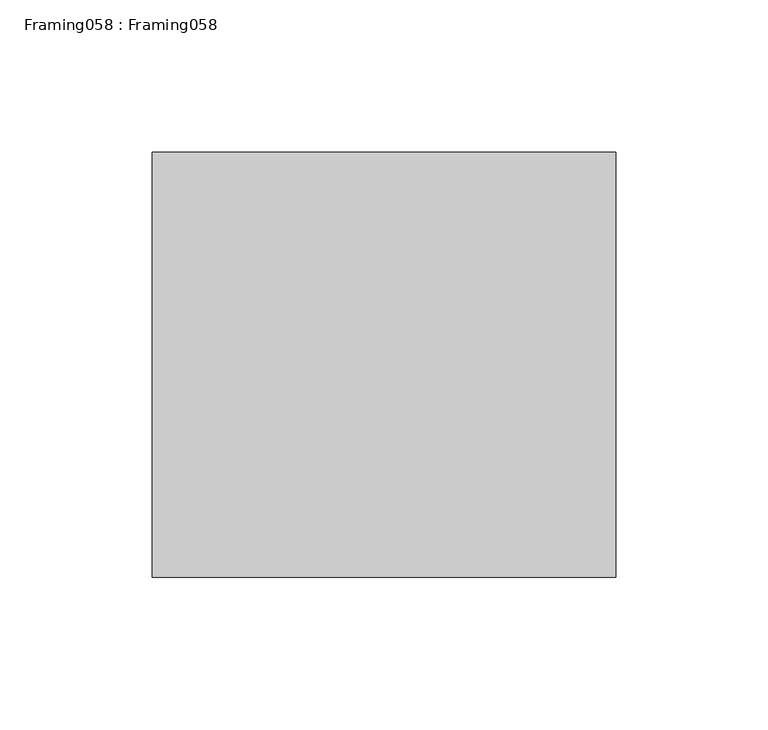
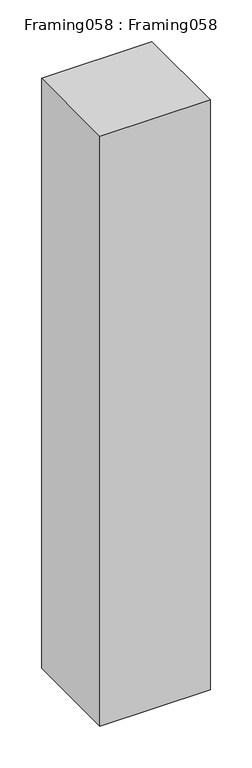
"""IFC4 building model written with IfcOpenShell, lengths in millimetres: proxy geometry, Framing058 : Framing058."""

from ifc_helpers import new_model, si_unit, frame, origin, place, context, project, spatial, polyline, outline, extrude, source, transform, mapped, element, save


def framing058_framing058_3deb3078(model_context):
    return source(origin(), model_context, "Body", "SweptSolid", [
        extrude(outline(polyline([(4475.0880859, 9730.3383229), (4475.0880859, 9590.6375834), (4322.6880859, 9590.6375834), (4322.6880859, 9730.3383229), (4475.0880859, 9730.3383229)])), frame((0.0, 0.0, 36582.096), z_axis=(0.0, 0.0, 1.0), x_axis=(1.0, 0.0, 0.0)), (0.0, 0.0, 1.0), 863.6),
    ])


if __name__ == "__main__":
    model = new_model("IFC4")
    model_context = context("Model", 3, world=origin())
    ifc_project = project(units=[si_unit("LENGTHUNIT", "METRE", prefix="MILLI")], contexts=[model_context])
    site = spatial("IfcSite", under=ifc_project)
    building = spatial("IfcBuilding", under=site)
    placement = place(None, origin())
    framing058_framing058_shape = framing058_framing058_3deb3078(model_context)
    element("IfcBuildingElementProxy", 1, Name="Framing058 : Framing058", ObjectType="Framing058 : Framing058", at=placement, inside=building, context=model_context, shape_type="MappedRepresentation", body=[
        mapped(framing058_framing058_shape, transform((0.0, 0.0, 0.0), x_axis=(1.0, 0.0, 0.0), y_axis=(0.0, 1.0, 0.0), z_axis=(0.0, 0.0, 1.0))),
    ])
    save(model, "model.ifc")

# Revit data of these elements
# Type "Framing058 : Framing058"
#   NameOverride = "Framing058"
# Element 1 (IfcBuildingElementProxy, "Framing058 : Framing058")
#   Materials on its faces: "WOOD FRAMING (SEE STRUCT DWGS)"
# Materials
#   "WOOD FRAMING (SEE STRUCT DWGS)": class "Unassigned", colour RGB 224 188 168, transparency 0, Cost = 0
